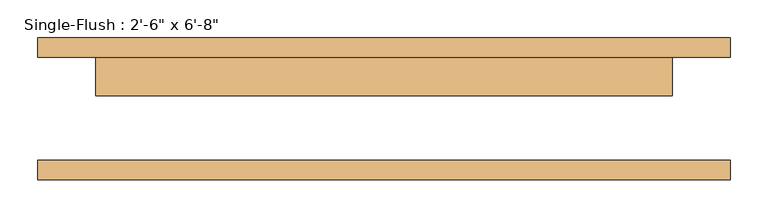
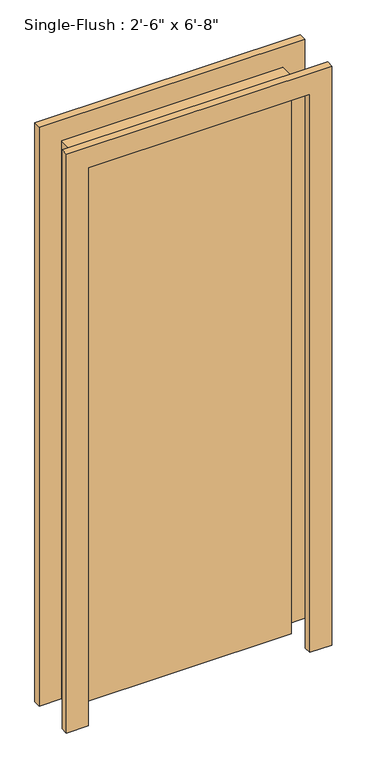
"""IFC4 building model written with IfcOpenShell, lengths in millimetres: door geometry."""

import ifcopenshell
import ifcopenshell.guid

model = None  # the IFC model being written
_history = None  # IfcOwnerHistory: only IFC2X3 demands one
_inside = {}  # id of a spatial element -> (the spatial element, [elements in it])
_under = {}  # id of a project, library or spatial element -> (it, [spatial elements below it])
_declared = {}  # id of a project -> (the project, [libraries it declares])
_typed = {}  # id of a type object -> (the type object, [elements of that type])
_made_of = {}  # id of a material, layer set ... -> (it, [elements and type objects made of it])


def new_model(schema):
    """Start an empty IFC model of exactly this schema.

    Asked for "IFC4X3", IfcOpenShell would pick the latest addendum, in which some entities
    have other attributes; the version numbers below select the first issue.
    IFC2X3 requires an IfcOwnerHistory on every rooted entity: one is made here for all.
    """
    global model, _history
    if schema == "IFC4X3":
        model = ifcopenshell.file(schema_version=(4, 3, 0, 0))
    else:
        model = ifcopenshell.file(schema=schema)
    _inside.clear()
    _under.clear()
    _declared.clear()
    _typed.clear()
    _made_of.clear()
    _history = None
    if model.schema == "IFC2X3":
        org = make("IfcOrganization", Name="unknown")
        user = make(
            "IfcPersonAndOrganization",
            ThePerson=make("IfcPerson", FamilyName="unknown"),
            TheOrganization=org,
        )
        app = make(
            "IfcApplication",
            ApplicationDeveloper=org,
            Version="unknown",
            ApplicationFullName="unknown",
            ApplicationIdentifier="unknown",
        )
        _history = make(
            "IfcOwnerHistory",
            OwningUser=user,
            OwningApplication=app,
            ChangeAction="ADDED",
            CreationDate=0,
        )
    return model


def make(cls, **values):
    """One entity of the class cls with the attributes given. An attribute that is None is left unset."""
    return model.create_entity(
        cls, **{name: value for name, value in values.items() if value is not None}
    )


def rooted(cls, **values):
    """An entity with a GlobalId (a new one), such as an element, a storey or a relation."""
    return make(cls, GlobalId=ifcopenshell.guid.new(), OwnerHistory=_history, **values)


def si_unit(unit_type, name, prefix=None):
    """IfcSIUnit, for example si_unit("LENGTHUNIT", "METRE", prefix="MILLI")."""
    return make("IfcSIUnit", UnitType=unit_type, Prefix=prefix, Name=name)


def assignment(units):
    """IfcUnitAssignment: the units of a project."""
    return None if units is None else make("IfcUnitAssignment", Units=units)


def point(xyz):
    """IfcCartesianPoint."""
    return None if xyz is None else make("IfcCartesianPoint", Coordinates=xyz)


def direction(xyz):
    """IfcDirection."""
    return None if xyz is None else make("IfcDirection", DirectionRatios=xyz)


def frame(location, z_axis=None, x_axis=None):
    """IfcAxis2Placement3D, a coordinate frame: its origin and axes. An axis left out is left unset."""
    return make(
        "IfcAxis2Placement3D",
        Location=point(location),
        Axis=direction(z_axis),
        RefDirection=direction(x_axis),
    )


def origin():
    """The frame at (0, 0, 0) with its axes left unset."""
    return frame((0.0, 0.0, 0.0))


def origin_with_axes():
    """The frame at (0, 0, 0) with the z axis (0, 0, 1) and the x axis (1, 0, 0) written out."""
    return frame((0.0, 0.0, 0.0), z_axis=(0.0, 0.0, 1.0), x_axis=(1.0, 0.0, 0.0))


def place(relative_to, where):
    """IfcLocalPlacement: puts the frame where relative to a parent placement (None: the world)."""
    return make(
        "IfcLocalPlacement", PlacementRelTo=relative_to, RelativePlacement=where
    )


def context(
    kind, dimensions, precision=None, world=None, true_north=None, identifier=None
):
    """IfcGeometricRepresentationContext, for example the 3D "Model" context."""
    return make(
        "IfcGeometricRepresentationContext",
        ContextIdentifier=identifier,
        ContextType=kind,
        CoordinateSpaceDimension=dimensions,
        Precision=precision,
        WorldCoordinateSystem=world,
        TrueNorth=true_north,
    )


def project(units=None, contexts=None):
    """IfcProject with its units and contexts."""
    return rooted(
        "IfcProject",
        Name="project",
        RepresentationContexts=contexts,
        UnitsInContext=assignment(units),
    )


def spatial(cls, under=None, at=None, **own):
    """A site, building, storey or space (cls), placed at a placement, below another one or the project."""
    s = rooted(cls, ObjectPlacement=at, **own)
    if under is not None:
        _under.setdefault(under.id(), (under, []))[1].append(s)
    return s


def polyline(points):
    """IfcPolyline through the points."""
    return make("IfcPolyline", Points=[point(p) for p in points])


def outline(outer, holes=None, kind="AREA"):
    """IfcArbitraryClosedProfileDef: a profile drawn as a closed curve; with holes, ...WithVoids."""
    if holes is None:
        return make("IfcArbitraryClosedProfileDef", ProfileType=kind, OuterCurve=outer)
    return make(
        "IfcArbitraryProfileDefWithVoids",
        ProfileType=kind,
        OuterCurve=outer,
        InnerCurves=holes,
    )


def extrude(swept, where, along, depth):
    """IfcExtrudedAreaSolid: the profile swept, set in the frame where, extruded along a direction by depth."""
    return make(
        "IfcExtrudedAreaSolid",
        SweptArea=swept,
        Position=where,
        ExtrudedDirection=direction(along),
        Depth=depth,
    )


def shape(context_of_items, identifier, shape_type, items):
    """IfcShapeRepresentation: the items that make up one representation, for example the "Body"."""
    return make(
        "IfcShapeRepresentation",
        ContextOfItems=context_of_items,
        RepresentationIdentifier=identifier,
        RepresentationType=shape_type,
        Items=items,
    )


def source(mapping_origin, context_of_items, identifier, shape_type, items):
    """IfcRepresentationMap: a shape defined once, which mapped items show again and again."""
    return make(
        "IfcRepresentationMap",
        MappingOrigin=mapping_origin,
        MappedRepresentation=shape(context_of_items, identifier, shape_type, items),
    )


def transform(
    local_origin,
    x_axis=None,
    y_axis=None,
    z_axis=None,
    scale=None,
    scale2=None,
    scale3=None,
    uniform=True,
):
    """IfcCartesianTransformationOperator3D, or its non-uniform kind. x_axis, y_axis, z_axis: its Axis1, 2, 3."""
    if uniform:
        return make(
            "IfcCartesianTransformationOperator3D",
            Axis1=direction(x_axis),
            Axis2=direction(y_axis),
            LocalOrigin=point(local_origin),
            Scale=scale,
            Axis3=direction(z_axis),
        )
    return make(
        "IfcCartesianTransformationOperator3DnonUniform",
        Axis1=direction(x_axis),
        Axis2=direction(y_axis),
        LocalOrigin=point(local_origin),
        Scale=scale,
        Axis3=direction(z_axis),
        Scale2=scale2,
        Scale3=scale3,
    )


def mapped(mapping_source, mapping_target):
    """IfcMappedItem: shows the shape of a source again, moved by a transform."""
    return make(
        "IfcMappedItem", MappingSource=mapping_source, MappingTarget=mapping_target
    )


def made_of(thing, what):
    """Note that an element or type object is made of a material, layer set ...; save() writes the relation."""
    if what is not None:
        _made_of.setdefault(what.id(), (what, []))[1].append(thing)
    return thing


def element(
    cls,
    number,
    at=None,
    inside=None,
    cuts=None,
    type_object=None,
    material=None,
    context=None,
    identifier="Body",
    shape_type=None,
    held_by="IfcProductDefinitionShape",
    body=None,
    shapes=None,
    **own,
):
    """One element of the class cls, such as IfcWall. Its Tag is "e" and its number.

    at: its placement. inside: the storey or other place that contains it. cuts: it is an
    opening in that element (IfcRelVoidsElement). A single representation is given by context,
    identifier, shape_type and body (its items); several are given by shapes. held_by: the class
    of the entity that holds the representations. save() writes the other relations.
    """
    e = rooted(cls, Tag="e%d" % number, ObjectPlacement=at, **own)
    if body is not None:
        shapes = [shape(context, identifier, shape_type, body)]
    if shapes is not None:
        e.Representation = make(held_by, Representations=shapes)
    if inside is not None:
        _inside.setdefault(inside.id(), (inside, []))[1].append(e)
    if cuts is not None:
        rooted(
            "IfcRelVoidsElement", RelatingBuildingElement=cuts, RelatedOpeningElement=e
        )
    if type_object is not None:
        _typed.setdefault(type_object.id(), (type_object, []))[1].append(e)
    return made_of(e, material)


def aggregate(whole, parts):
    """IfcRelAggregates: a whole, such as a stair, and the parts it consists of."""
    return rooted("IfcRelAggregates", RelatingObject=whole, RelatedObjects=parts)


def save(model, path):
    """Write the relations noted so far, then the file.

    IfcRelAggregates (storeys below a building ...), IfcRelContainedInSpatialStructure (elements
    in a storey), IfcRelDefinesByType, IfcRelAssociatesMaterial and IfcRelDeclares: one each for
    every whole, place, type object, material and project.
    """
    for whole, parts in _under.values():
        aggregate(whole, parts)
    for where, things in _inside.values():
        rooted(
            "IfcRelContainedInSpatialStructure",
            RelatedElements=things,
            RelatingStructure=where,
        )
    for kind, things in _typed.values():
        rooted("IfcRelDefinesByType", RelatedObjects=things, RelatingType=kind)
    for what, things in _made_of.values():
        rooted("IfcRelAssociatesMaterial", RelatedObjects=things, RelatingMaterial=what)
    for by, libraries in _declared.values():
        rooted("IfcRelDeclares", RelatingContext=by, RelatedDefinitions=libraries)
    model.write(path)


def door_0b154108(model_context):
    return source(origin(), model_context, "Body", "SweptSolid", [
        extrude(outline(polyline([(2108.2, -457.2), (0.0, -457.2), (0.0, -381.0), (2032.0, -381.0), (2032.0, 381.0), (0.0, 381.0), (0.0, 457.2), (2108.2, 457.2), (2108.2, -457.2)])), frame((0.0, 68.2625, 0.0), z_axis=(0.0, 1.0, 0.0), x_axis=(0.0, 0.0, 1.0)), (0.0, 0.0, 1.0), 25.4),
        extrude(outline(polyline([(2108.2, 457.2), (2108.2, -457.2), (0.0, -457.2), (0.0, -381.0), (2032.0, -381.0), (2032.0, 381.0), (0.0, 381.0), (0.0, 457.2), (2108.2, 457.2)])), frame((0.0, -93.6625, 0.0), z_axis=(0.0, 1.0, 0.0), x_axis=(0.0, 0.0, 1.0)), (0.0, 0.0, 1.0), 25.4),
        extrude(outline(polyline([(381.0, 17.4625), (-381.0, 17.4625), (-381.0, 68.2625), (381.0, 68.2625), (381.0, 17.4625)])), origin_with_axes(), (0.0, 0.0, 1.0), 2032.0),
    ])


if __name__ == "__main__":
    model = new_model("IFC4")
    model_context = context("Model", 3, world=origin())
    ifc_project = project(units=[si_unit("LENGTHUNIT", "METRE", prefix="MILLI")], contexts=[model_context])
    site = spatial("IfcSite", under=ifc_project)
    building = spatial("IfcBuilding", under=site)
    placement = place(None, origin())
    door_shape = door_0b154108(model_context)
    element("IfcDoor", 1, ObjectType="Single-Flush : 2'-6\" x 6'-8\"", at=placement, inside=building, context=model_context, shape_type="MappedRepresentation", body=[
        mapped(door_shape, transform((0.0, 0.0, 0.0), x_axis=(1.0, 0.0, 0.0), y_axis=(0.0, 1.0, 0.0), z_axis=(0.0, 0.0, 1.0))),
    ])
    save(model, "model.ifc")

# Revit data of these elements
# Type "Single-Flush : 2'-6\" x 6'-8\""
#   Type Mark = "13"
#   Construction Type Id = "MDOOR"
#   Assembly Code = "C1020"
#   Analytic Construction = "Metal"
#   Thickness = 0' - 2"
#   Heat Transfer Coefficient (U) = 3.7021 W/(m²·K)
#   Height = 6' - 8"
#   Trim Projection Ext = 0' - 1"
#   Trim Projection Int = 0' - 1"
#   Trim Width = 0' - 3"
#   Width = 2' - 6"
#   Door Material = Door - Panel
#   Frame Material = Door - Frame
#   Visual Light Transmittance = 0
#   Solar Heat Gain Coefficient = 0
#   Function = (empty or 0)
#   Wall Closure = (empty or 0)
# Element 1 (IfcDoor, "Single-Flush : 2'-6\" x 6'-8\"")
#   Materials on its faces: "Door - Frame", "Door - Panel"
# Materials
#   "Door - Panel": class "Wood", colour RGB 210 159 95, transparency 0, Cost = 0
#   "Door - Frame": class "Miscellaneous", colour RGB 118 70 51, transparency 0, Cost = 0
